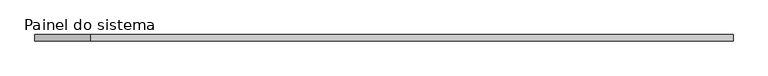
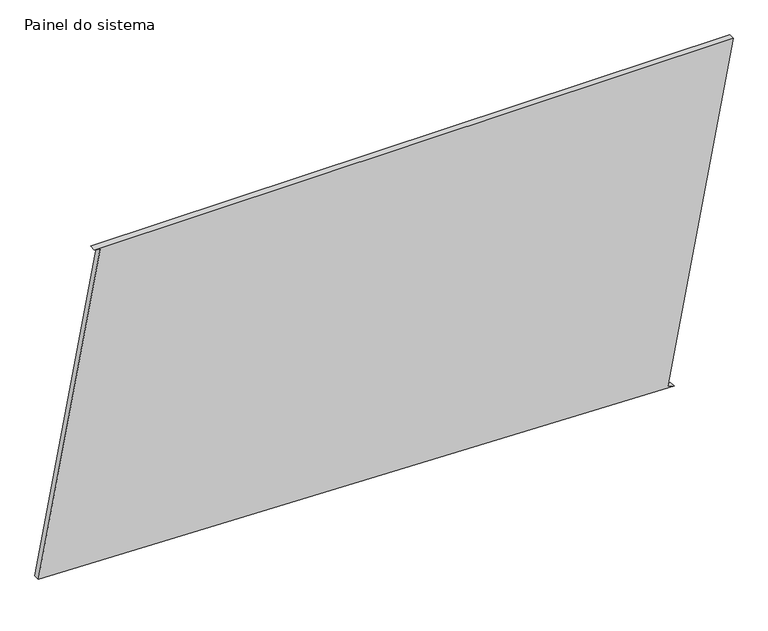
"""IFC4 building model written with IfcOpenShell, lengths in millimetres: plate geometry, Painel do sistema : Envidraçado."""

from ifc_helpers import new_model, si_unit, frame, origin, place, context, project, spatial, polyline, outline, extrude, source, transform, mapped, element, save


def painel_do_sistema_66235948(model_context):
    return source(origin(), model_context, "Body", "SweptSolid", [
        extrude(outline(polyline([(0.0, 1169.5659801), (4.6288169, 1144.998236), (1407.2008072, 1409.2572936), (1407.2008072, -1183.1957613), (1402.5719903, -1158.6280171), (72.3409423, -1409.2572936), (0.0, 1169.5659801)])), frame((0.0, 24.5, 0.0), z_axis=(0.0, 1.0, 0.0), x_axis=(0.0, 0.0, 1.0)), (0.0, 0.0, 1.0), 25.0),
    ])


if __name__ == "__main__":
    model = new_model("IFC4")
    model_context = context("Model", 3, world=origin())
    ifc_project = project(units=[si_unit("LENGTHUNIT", "METRE", prefix="MILLI")], contexts=[model_context])
    site = spatial("IfcSite", under=ifc_project)
    building = spatial("IfcBuilding", under=site)
    placement = place(None, origin())
    painel_do_sistema_shape = painel_do_sistema_66235948(model_context)
    element("IfcPlate", 1, ObjectType="Painel do sistema : Envidraçado", at=placement, inside=building, context=model_context, shape_type="MappedRepresentation", body=[
        mapped(painel_do_sistema_shape, transform((0.0, 0.0, 0.0), x_axis=(1.0, 0.0, 0.0), y_axis=(0.0, 1.0, 0.0), z_axis=(0.0, 0.0, 1.0))),
    ])
    save(model, "model.ifc")

# Revit data of these elements
# Type "Painel do sistema : Envidraçado"
#   Construction Type Id = "GSP4R"
#   Analytic Construction = "Vidraça única Pilkington 1/8 pol"
#   Visual Light Transmittance = 0.9
#   Solar Heat Gain Coefficient = 0.86
#   Heat Transfer Coefficient (U) = 6.7069 W/(m²·K)
# Element 1 (IfcPlate, "Painel do sistema : Envidraçado")
#   Materials on its faces: "Vidro"
# Materials
#   "Vidro": class "Vidro", colour RGB 0 128 192, transparency 0.9, Description = "Vidro de sílica", Cost = 0
